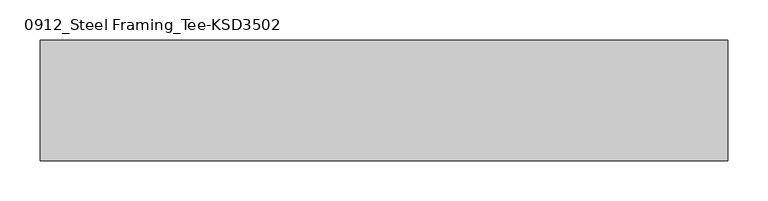
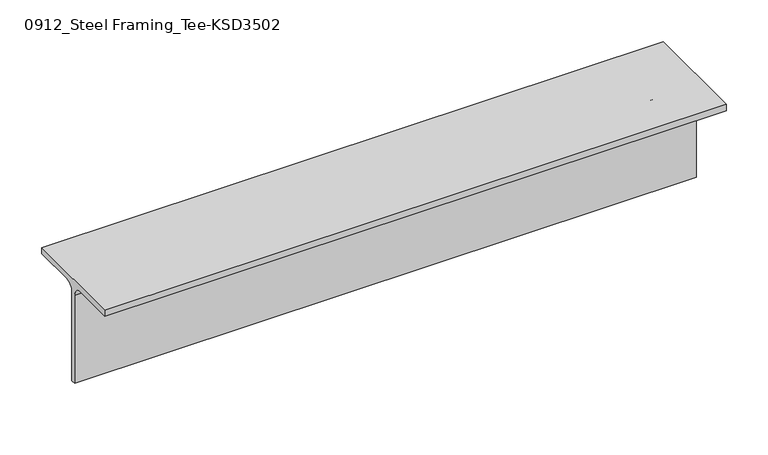
"""IFC4 building model written with IfcOpenShell, lengths in millimetres: member geometry, 0912_Steel Framing_Tee-KSD3502 : H_SB_ASB_CT-150x150x6.5x9."""

from ifc_helpers import new_model, si_unit, point, frame, frame_2d, origin, place, context, project, spatial, polyline, circle_curve, trimmed, segment, composite_curve, outline, extrude, source, transform, mapped, element, save


def member_0912_steel_framing_tee_ksd3502_8ca30748(model_context):
    return source(origin(), model_context, "Body", "SweptSolid", [
        extrude(outline(composite_curve([segment(polyline([(-75.0, 75.0), (75.0, 75.0), (75.0, 66.0), (16.25, 66.0)]), True, "CONTINUOUS"), segment(trimmed(circle_curve(frame_2d((16.25, 53.0)), 13.0), [point((16.25, 66.0))], [point((3.25, 53.0))], True, "CARTESIAN"), True, "CONTINUOUS"), segment(polyline([(3.25, 53.0), (3.25, -75.0), (-3.25, -75.0), (-3.25, 53.0)]), True, "CONTINUOUS"), segment(trimmed(circle_curve(frame_2d((-16.25, 53.0)), 13.0), [point((-3.25, 53.0))], [point((-16.25, 66.0))], True, "CARTESIAN"), True, "CONTINUOUS"), segment(polyline([(-16.25, 66.0), (-75.0, 66.0), (-75.0, 75.0)]), True, "CONTINUOUS")], self_intersect=False)), frame((-500.0, 0.0, 0.0), z_axis=(1.0, 0.0, 0.0), x_axis=(0.0, 1.0, 0.0)), (0.0, 0.0, 1.0), 856.1),
    ])


if __name__ == "__main__":
    model = new_model("IFC4")
    model_context = context("Model", 3, world=origin())
    ifc_project = project(units=[si_unit("LENGTHUNIT", "METRE", prefix="MILLI")], contexts=[model_context])
    site = spatial("IfcSite", under=ifc_project)
    building = spatial("IfcBuilding", under=site)
    placement = place(None, origin())
    member_0912_steel_framing_tee_ksd3502_shape = member_0912_steel_framing_tee_ksd3502_8ca30748(model_context)
    element("IfcMember", 1, ObjectType="0912_Steel Framing_Tee-KSD3502 : H_SB_ASB_CT-150x150x6.5x9", at=placement, inside=building, context=model_context, shape_type="MappedRepresentation", body=[
        mapped(member_0912_steel_framing_tee_ksd3502_shape, transform((0.0, 0.0, 0.0), x_axis=(1.0, 0.0, 0.0), y_axis=(0.0, 1.0, 0.0), z_axis=(0.0, 0.0, 1.0))),
    ])
    save(model, "model.ifc")

# Revit data of these elements
# Type "0912_Steel Framing_Tee-KSD3502 : H_SB_ASB_CT-150x150x6.5x9"
#   H_WM Code_1 = "S01AA003-00001 | Main Steel Structure Fabrication Work | Shelter/Building | Light Steel - Standard (30KG/M>Weight) | Material: (   )"
#   H_WM Code_2 = "S03AA029-00001 | Main Steel Structure Erection Work | Shelter/Building | Light Steel (30KG/M>Weight) | Material: (   )"
#   H_WM Code_3 = "S01AA010-00001 | Main Steel Structure Fabrication Work | Shelter/Building | Steel Painting/Coating | for Non-Fireproofed Steel Surface, Surface Preparation, Primer, Second & Final Coat | Material: (   )"
#   H_Q'ty Cal Type Tag = "SB-Q2"
#   Width = 15.0 cm
#   Web Thickness = 0.65 cm
#   Web Fillet = 1.3 cm
#   Section Area = 23.39 cm²
#   Perimeter = 0.60 m²/m
#   Nominal Weight = 18.40 kgf/m
#   Height = 15.0 cm
#   Flange Thickness = 0.9 cm
#   Centroid Vertical = 7.5 cm
#   Centroid Horizontal = 7.5 cm
#   Length [instance default] = 1.5000 m
#   Structural Material [instance default] = Steel, 45-345
#   Warping Constant = (empty or 0)
#   Torsional Moment of Inertia = 0
#   Section Name Key = ""
#   Plastic Modulus weak axis = 0
#   Plastic Modulus strong axis = 0
#   Moment of Inertia weak axis = 0
#   Moment of Inertia strong axis = 0
#   Elastic Modulus weak axis = 0
#   Elastic Modulus strong axis = 0
#   Bolt Spacing = 0
#   Assembly Code = ""
# Element 1 (IfcMember, "0912_Steel Framing_Tee-KSD3502 : H_SB_ASB_CT-150x150x6.5x9")
#   Structural Material = none
# Materials
#   "Steel, 45-345": class "Metal", colour RGB 189 187 185, transparency 0, Description = "Steel 345 MPa", Cost = 0
